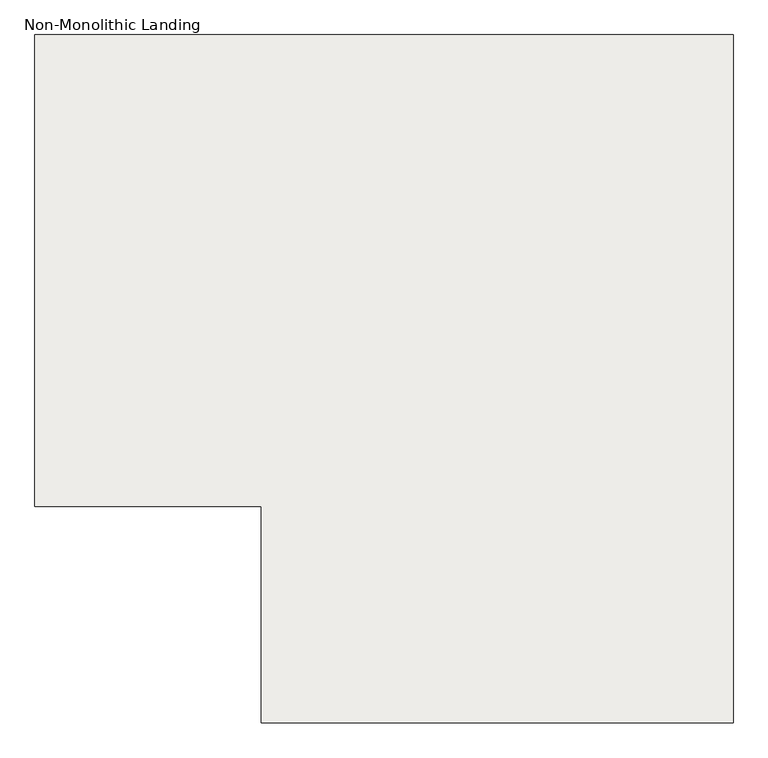
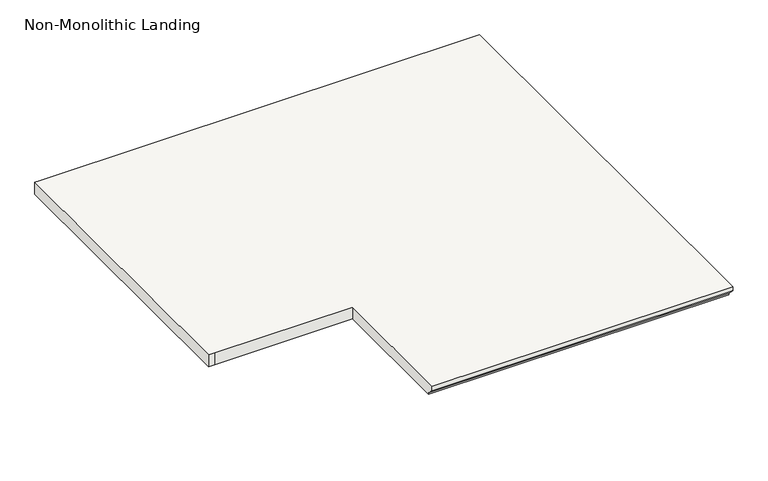
"""IFC4 building model written with IfcOpenShell, lengths in millimetres: slab geometry, Non-Monolithic Landing."""

from ifc_helpers import new_model, si_unit, origin, place, context, project, spatial, faceted_brep, source, transform, mapped, element, save


def non_monolithic_landing_afb1a1ec(model_context):
    return source(origin(), model_context, "Body", "Brep", [
        faceted_brep([(-3020.5507921, -4668.4601743, 1200.15), (-3020.5507921, -4668.4601743, 1219.2), (-4239.7507921, -4668.4601743, 1219.2), (-4239.7507921, -4668.4601743, 1200.15), (-3020.5507921, -4643.0601743, 1174.75), (-4239.7507921, -4643.0601743, 1174.75), (-3020.5507921, -2890.4601743, 1219.2), (-4798.5507921, -2890.4601743, 1219.2), (-4823.9507921, -2890.4601743, 1219.2), (-4823.9507921, -4109.6601743, 1219.2), (-4798.5507921, -4109.6601743, 1219.2), (-4239.7507921, -4109.6601743, 1219.2), (-3020.5507921, -4643.0601743, 1168.4), (-4239.7507921, -4643.0601743, 1168.4), (-4239.7507921, -4109.6601743, 1168.4), (-4798.5507921, -4109.6601743, 1168.4), (-4823.9507921, -4109.6601743, 1168.4), (-4823.9507921, -2890.4601743, 1168.4), (-4798.5507921, -2890.4601743, 1168.4), (-3020.5507921, -2890.4601743, 1168.4)], [[[0, 1, 2, 3]], [[4, 0, 3, 5]], [[6, 7, 8, 9, 10, 11, 2, 1]], [[12, 13, 14, 15, 16, 17, 18, 19]], [[13, 12, 4, 5]], [[6, 1, 0, 4, 12, 19]], [[7, 6, 19, 18]], [[8, 7, 18, 17]], [[9, 8, 17, 16]], [[10, 9, 16, 15]], [[11, 10, 15, 14]], [[2, 11, 14, 13, 5, 3]]]),
    ])


if __name__ == "__main__":
    model = new_model("IFC4")
    model_context = context("Model", 3, world=origin())
    ifc_project = project(units=[si_unit("LENGTHUNIT", "METRE", prefix="MILLI")], contexts=[model_context])
    site = spatial("IfcSite", under=ifc_project)
    building = spatial("IfcBuilding", under=site)
    placement = place(None, origin())
    non_monolithic_landing_shape = non_monolithic_landing_afb1a1ec(model_context)
    element("IfcSlab", 1, ObjectType="Non-Monolithic Landing", at=placement, inside=building, context=model_context, shape_type="MappedRepresentation", body=[
        mapped(non_monolithic_landing_shape, transform((0.0, 0.0, 0.0), x_axis=(1.0, 0.0, 0.0), y_axis=(0.0, 1.0, 0.0), z_axis=(0.0, 0.0, 1.0))),
    ])
    save(model, "model.ifc")
